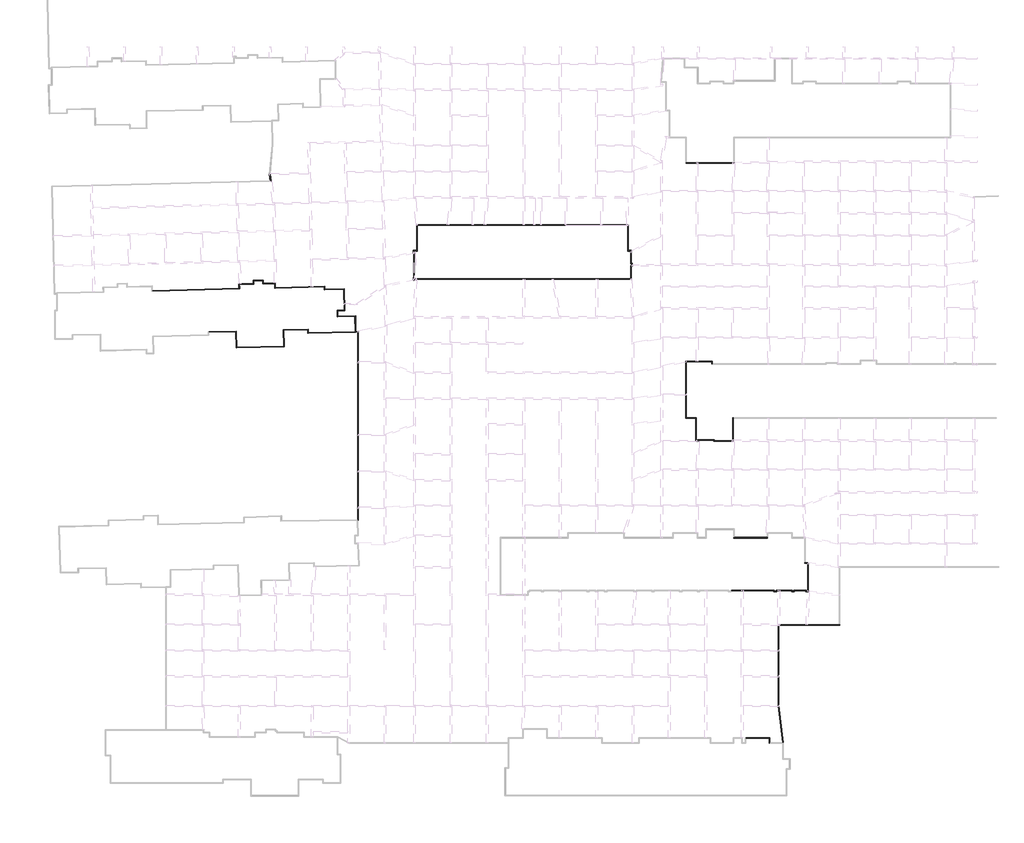
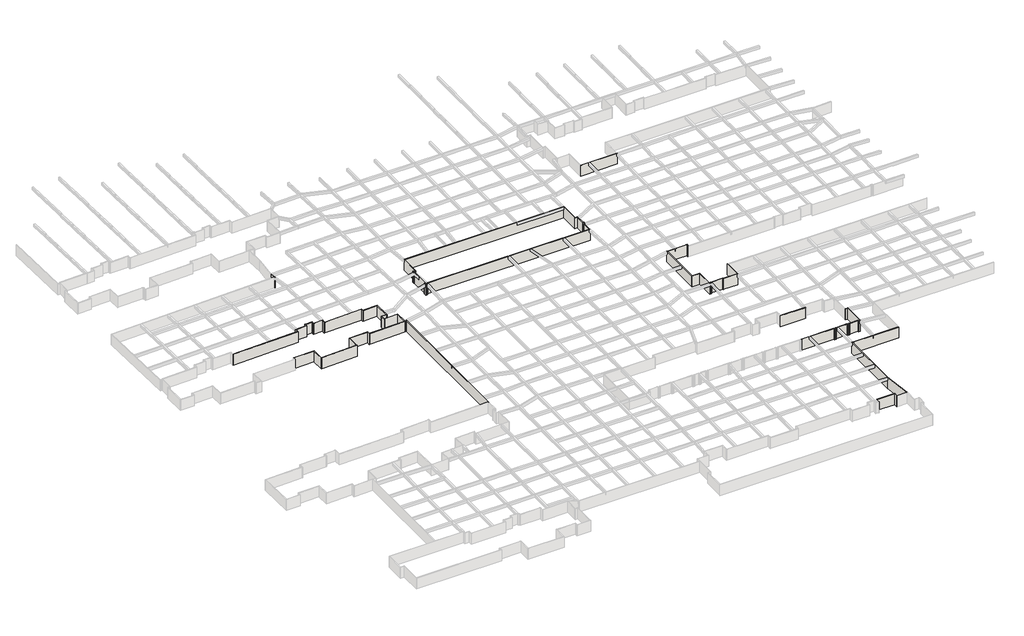
# One storey, part 4 of 20: 75 walls.
"""IFC4 building model written with IfcOpenShell, lengths in millimetres."""

from ifc_helpers import new_model, si_unit, origin, origin_with_axes, place, context, project, spatial, polyline, outline, extrude, faceted_brep, element, save

model = new_model("IFC4")

# Units and contexts
model_context = context("Model", 3, world=origin())
ifc_project = project(units=[si_unit("LENGTHUNIT", "METRE", prefix="MILLI")], contexts=[model_context])

# Site, building, storey
site = spatial("IfcSite", under=ifc_project)
building = spatial("IfcBuilding", under=site)
storey = spatial("IfcBuildingStorey", under=building, Name="户型图", Elevation=0.0)

# Walls
placement = place(None, origin())
element("IfcWall", 1, ObjectType="所有墙体", at=placement, inside=storey, context=model_context, shape_type="Brep", body=[
    faceted_brep([(22764.2529371, 124971.3529529, 0.0), (22969.277881, 123512.5246746, 0.0), (22986.0907128, 123392.8951605, 0.0), (22986.0907128, 123392.8951605, 3300.0), (22969.277881, 123512.5246746, 3300.0), (22764.2529371, 124971.3529529, 3300.0), (22884.987918, 124974.5145097, 0.0), (22884.987918, 124974.5145097, 3300.0), (23106.8607981, 123395.8069362, 3300.0), (23106.8607981, 123395.8069362, 0.0)], [[[0, 1, 2, 3, 4, 5]], [[6, 7, 8, 9]], [[2, 1, 0, 6, 9]], [[5, 4, 3, 8, 7]], [[0, 5, 7, 6]], [[3, 2, 9, 8]]]),
])
element("IfcWall", 2, ObjectType="所有墙体", at=placement, inside=storey, context=model_context, shape_type="Brep", body=[
    faceted_brep([(9470.1632227, 90251.8005582, 0.0), (15349.8840277, 90393.5386622, 0.0), (15469.8491762, 90396.4305738, 0.0), (15469.8491762, 90396.4305738, 3300.0), (15349.8840277, 90393.5386622, 3300.0), (9470.1632227, 90251.8005582, 3300.0), (9470.1632227, 90371.8354198, 0.0), (9470.1632227, 90371.8354198, 3300.0), (15466.9572646, 90516.3957223, 3300.0), (15466.9572646, 90516.3957223, 0.0)], [[[0, 1, 2, 3, 4, 5]], [[6, 7, 8, 9]], [[2, 1, 0, 6, 9]], [[5, 4, 3, 8, 7]], [[0, 5, 7, 6]], [[3, 2, 9, 8]]]),
])
element("IfcWall", 3, ObjectType="所有墙体", at=placement, inside=storey, context=model_context, shape_type="Brep", body=[
    faceted_brep([(15349.8840277, 90393.5386622, 0.0), (15435.7681225, 86830.8093449, 0.0), (15435.7681225, 86830.8093449, 3300.0), (15349.8840277, 90393.5386622, 3300.0), (15469.8491762, 90396.4305738, 0.0), (15469.8491762, 90396.4305738, 3300.0), (15552.8413594, 86953.6664049, 3300.0), (15555.7332709, 86833.7012564, 3300.0), (15555.7332709, 86833.7012564, 0.0), (15552.8413594, 86953.6664049, 0.0)], [[[0, 1, 2, 3]], [[4, 5, 6, 7, 8, 9]], [[1, 0, 4, 9, 8]], [[3, 2, 7, 6, 5]], [[0, 3, 5, 4]], [[2, 1, 8, 7]]]),
])
element("IfcWall", 4, ObjectType="所有墙体", at=placement, inside=storey, context=model_context, shape_type="Brep", body=[
    faceted_brep([(15555.7332709, 86833.7012564, 0.0), (25984.4133708, 87085.0977757, 0.0), (25984.4133708, 87085.0977757, 3300.0), (15555.7332709, 86833.7012564, 3300.0), (15552.8413594, 86953.6664049, 0.0), (15552.8413594, 86953.6664049, 3300.0), (25861.5563108, 87202.1710126, 3300.0), (25981.5214593, 87205.0629242, 3300.0), (25981.5214593, 87205.0629242, 0.0), (25861.5563108, 87202.1710126, 0.0)], [[[0, 1, 2, 3]], [[4, 5, 6, 7, 8, 9]], [[1, 0, 4, 9, 8]], [[3, 2, 7, 6, 5]], [[0, 3, 5, 4]], [[2, 1, 8, 7]]]),
])
element("IfcWall", 5, ObjectType="所有墙体", at=placement, inside=storey, context=model_context, shape_type="Brep", body=[
    faceted_brep([(25981.5214593, 87205.0629242, 0.0), (25898.5292761, 90647.8270931, 0.0), (25895.6373645, 90767.7922416, 0.0), (25895.6373645, 90767.7922416, 3300.0), (25898.5292761, 90647.8270931, 3300.0), (25981.5214593, 87205.0629242, 3300.0), (25861.5563108, 87202.1710126, 0.0), (25861.5563108, 87202.1710126, 3300.0), (25775.6722161, 90764.90033, 3300.0), (25775.6722161, 90764.90033, 0.0)], [[[0, 1, 2, 3, 4, 5]], [[6, 7, 8, 9]], [[2, 1, 0, 6, 9]], [[5, 4, 3, 8, 7]], [[0, 5, 7, 6]], [[3, 2, 9, 8]]]),
])
element("IfcWall", 6, ObjectType="所有墙体", at=placement, inside=storey, context=model_context, shape_type="Brep", body=[
    faceted_brep([(25898.5292761, 90647.8270931, 0.0), (31175.86669, 90775.0439838, 0.0), (31295.86669, 90777.9367356, 0.0), (31295.86669, 90777.9367356, 3300.0), (31175.86669, 90775.0439838, 3300.0), (25898.5292761, 90647.8270931, 3300.0), (25895.6373645, 90767.7922416, 0.0), (25895.6373645, 90767.7922416, 3300.0), (31295.86669, 90897.9715972, 3300.0), (31295.86669, 90897.9715972, 0.0)], [[[0, 1, 2, 3, 4, 5]], [[6, 7, 8, 9]], [[2, 1, 0, 6, 9]], [[5, 4, 3, 8, 7]], [[0, 5, 7, 6]], [[3, 2, 9, 8]]]),
])
element("IfcWall", 7, ObjectType="所有墙体", at=placement, inside=storey, context=model_context, shape_type="Brep", body=[
    faceted_brep([(31175.86669, 90775.0439838, 0.0), (31175.86669, 89975.0439838, 0.0), (31175.86669, 89975.0439838, 3300.0), (31175.86669, 90775.0439838, 3300.0), (31295.86669, 90777.9367356, 0.0), (31295.86669, 90777.9367356, 3300.0), (31295.86669, 90097.9715972, 3300.0), (31295.86669, 89977.9367356, 3300.0), (31295.86669, 89977.9367356, 0.0), (31295.86669, 90097.9715972, 0.0)], [[[0, 1, 2, 3]], [[4, 5, 6, 7, 8, 9]], [[1, 0, 4, 9, 8]], [[3, 2, 7, 6, 5]], [[0, 3, 5, 4]], [[2, 1, 8, 7]]]),
])
element("IfcWall", 8, ObjectType="所有墙体", at=placement, inside=storey, context=model_context, shape_type="SweptSolid", body=[
    extrude(outline(polyline([(41741.4257555, 90229.7401437), (31295.86669, 89977.9367356), (31295.86669, 90097.9715972), (41724.2086067, 90349.3599642), (41741.4257555, 90229.7401437)])), origin_with_axes(), (0.0, 0.0, 1.0), 3300.0),
])
element("IfcWall", 9, ObjectType="所有墙体", at=placement, inside=storey, context=model_context, shape_type="Brep", body=[
    faceted_brep([(41741.4257555, 90229.7401437, 0.0), (42190.0, 90349.9352502, 0.0), (42310.0, 90382.0891533, 0.0), (42310.0, 90382.0891533, 3300.0), (42190.0, 90349.9352502, 3300.0), (41741.4257555, 90229.7401437, 3300.0), (41724.2086067, 90349.3599642, 0.0), (41724.2086067, 90349.3599642, 3300.0), (42310.0, 90506.322295, 3300.0), (42310.0, 90506.322295, 0.0)], [[[0, 1, 2, 3, 4, 5]], [[6, 7, 8, 9]], [[2, 1, 0, 6, 9]], [[5, 4, 3, 8, 7]], [[0, 5, 7, 6]], [[3, 2, 9, 8]]]),
])
element("IfcWall", 10, ObjectType="所有墙体", at=placement, inside=storey, context=model_context, shape_type="Brep", body=[
    faceted_brep([(42190.0, 90349.9352502, 0.0), (42190.0, 49087.0906084, 0.0), (42190.0, 48967.072329, 0.0), (42190.0, 48967.072329, 3300.0), (42190.0, 49087.0906084, 3300.0), (42190.0, 90349.9352502, 3300.0), (42310.0, 90382.0891533, 0.0), (42310.0, 90382.0891533, 3300.0), (42310.0, 48969.1669368, 3300.0), (42310.0, 48969.1669368, 0.0)], [[[0, 1, 2, 3, 4, 5]], [[6, 7, 8, 9]], [[2, 1, 0, 6, 9]], [[5, 4, 3, 8, 7]], [[0, 5, 7, 6]], [[3, 2, 9, 8]]]),
])
element("IfcWall", 11, ObjectType="所有墙体", at=placement, inside=storey, context=model_context, shape_type="Brep", body=[
    faceted_brep([(127432.0, 1046.0, 0.0), (132562.0, 1046.0, 0.0), (132682.0, 1046.0, 0.0), (132682.0, 1046.0, 3300.0), (132562.0, 1046.0, 3300.0), (127432.0, 1046.0, 3300.0), (127432.0, 1166.0, 0.0), (127432.0, 1166.0, 3300.0), (132682.0, 1166.0, 3300.0), (132682.0, 1166.0, 0.0)], [[[0, 1, 2, 3, 4, 5]], [[6, 7, 8, 9]], [[2, 1, 0, 6, 9]], [[5, 4, 3, 8, 7]], [[0, 5, 7, 6]], [[3, 2, 9, 8]]]),
])
element("IfcWall", 12, ObjectType="所有墙体", at=placement, inside=storey, context=model_context, shape_type="Brep", body=[
    faceted_brep([(132562.0, 1046.0, 0.0), (132562.0, -63.5203758, 0.0), (132562.0, -63.5203758, 3300.0), (132562.0, 1046.0, 3300.0), (132682.0, 1046.0, 0.0), (132682.0, 1046.0, 3300.0), (132682.0, 56.4796242, 3300.0), (132682.0, -63.5203758, 3300.0), (132682.0, -63.5203758, 0.0), (132682.0, 56.4796242, 0.0)], [[[0, 1, 2, 3]], [[4, 5, 6, 7, 8, 9]], [[1, 0, 4, 9, 8]], [[3, 2, 7, 6, 5]], [[0, 3, 5, 4]], [[2, 1, 8, 7]]]),
])
element("IfcWall", 13, ObjectType="所有墙体", at=placement, inside=storey, context=model_context, shape_type="SweptSolid", body=[
    extrude(outline(polyline([(134683.7348611, 8238.28244), (135688.3339273, 56.4796242), (135567.4327482, 56.4796242), (134563.7348611, 8230.9429256), (134683.7348611, 8238.28244)])), origin_with_axes(), (0.0, 0.0, 1.0), 3300.0),
])
element("IfcWall", 14, ObjectType="所有墙体", at=placement, inside=storey, context=model_context, shape_type="Brep", body=[
    faceted_brep([(134683.7348611, 8238.28244, 0.0), (134683.7348611, 25874.6126828, 0.0), (134683.7348611, 25994.6126828, 0.0), (134683.7348611, 25994.6126828, 3300.0), (134683.7348611, 25874.6126828, 3300.0), (134683.7348611, 8238.28244, 3300.0), (134563.7348611, 8230.9429256, 0.0), (134563.7348611, 8230.9429256, 3300.0), (134563.7348611, 25994.6126828, 3300.0), (134563.7348611, 25994.6126828, 0.0)], [[[0, 1, 2, 3, 4, 5]], [[6, 7, 8, 9]], [[2, 1, 0, 6, 9]], [[5, 4, 3, 8, 7]], [[0, 5, 7, 6]], [[3, 2, 9, 8]]]),
])
element("IfcWall", 15, ObjectType="所有墙体", at=placement, inside=storey, context=model_context, shape_type="Brep", body=[
    faceted_brep([(134683.7348611, 25874.6126828, 0.0), (148100.0, 25874.6126828, 0.0), (148100.0, 25874.6126828, 3300.0), (134683.7348611, 25874.6126828, 3300.0), (134683.7348611, 25994.6126828, 0.0), (134683.7348611, 25994.6126828, 3300.0), (147980.0, 25994.6126828, 3300.0), (148100.0, 25994.6126828, 3300.0), (148100.0, 25994.6126828, 0.0), (147980.0, 25994.6126828, 0.0)], [[[0, 1, 2, 3]], [[4, 5, 6, 7, 8, 9]], [[1, 0, 4, 9, 8]], [[3, 2, 7, 6, 5]], [[0, 3, 5, 4]], [[2, 1, 8, 7]]]),
])
element("IfcWall", 16, ObjectType="所有墙体", at=placement, inside=storey, context=model_context, shape_type="Brep", body=[
    faceted_brep([(114310.0, 127379.0, 0.0), (124860.0, 127379.0, 0.0), (124860.0, 127379.0, 3300.0), (114310.0, 127379.0, 3300.0), (114310.0, 127499.0, 0.0), (114310.0, 127499.0, 3300.0), (124740.0, 127499.0, 3300.0), (124860.0, 127499.0, 3300.0), (124860.0, 127499.0, 0.0), (124740.0, 127499.0, 0.0)], [[[0, 1, 2, 3]], [[4, 5, 6, 7, 8, 9]], [[1, 0, 4, 9, 8]], [[3, 2, 7, 6, 5]], [[0, 3, 5, 4]], [[2, 1, 8, 7]]]),
])
element("IfcWall", 17, ObjectType="所有墙体", at=placement, inside=storey, context=model_context, shape_type="Brep", body=[
    faceted_brep([(114224.0, 83917.0, 0.0), (114224.0, 71310.0, 0.0), (114224.0, 71310.0, 3300.0), (114224.0, 83917.0, 3300.0), (114344.0, 83917.0, 0.0), (114344.0, 83917.0, 3300.0), (114344.0, 83797.0, 3300.0), (114344.0, 71430.0, 3300.0), (114344.0, 71310.0, 3300.0), (114344.0, 71310.0, 0.0), (114344.0, 71430.0, 0.0), (114344.0, 83797.0, 0.0)], [[[0, 1, 2, 3]], [[4, 5, 6, 7, 8, 9, 10, 11]], [[1, 0, 4, 11, 10, 9]], [[3, 2, 8, 7, 6, 5]], [[2, 1, 9, 8]], [[0, 3, 5, 4]]]),
])
element("IfcWall", 18, ObjectType="所有墙体", at=placement, inside=storey, context=model_context, shape_type="Brep", body=[
    faceted_brep([(114344.0, 71310.0, 0.0), (116431.0, 71310.0, 0.0), (116551.0, 71310.0, 0.0), (116551.0, 71310.0, 3300.0), (116431.0, 71310.0, 3300.0), (114344.0, 71310.0, 3300.0), (114344.0, 71430.0, 0.0), (114344.0, 71430.0, 3300.0), (116551.0, 71430.0, 3300.0), (116551.0, 71430.0, 0.0)], [[[0, 1, 2, 3, 4, 5]], [[6, 7, 8, 9]], [[2, 1, 0, 6, 9]], [[5, 4, 3, 8, 7]], [[0, 5, 7, 6]], [[3, 2, 9, 8]]]),
])
element("IfcWall", 19, ObjectType="所有墙体", at=placement, inside=storey, context=model_context, shape_type="Brep", body=[
    faceted_brep([(116431.0, 71310.0, 0.0), (116431.0, 66283.0, 0.0), (116431.0, 66283.0, 3300.0), (116431.0, 71310.0, 3300.0), (116551.0, 71310.0, 0.0), (116551.0, 71310.0, 3300.0), (116551.0, 66403.0, 3300.0), (116551.0, 66283.0, 3300.0), (116551.0, 66283.0, 0.0), (116551.0, 66403.0, 0.0)], [[[0, 1, 2, 3]], [[4, 5, 6, 7, 8, 9]], [[1, 0, 4, 9, 8]], [[3, 2, 7, 6, 5]], [[0, 3, 5, 4]], [[2, 1, 8, 7]]]),
])
element("IfcWall", 20, ObjectType="所有墙体", at=placement, inside=storey, context=model_context, shape_type="SweptSolid", body=[
    extrude(outline(polyline([(116917.0, 66283.0), (116551.0, 66283.0), (116551.0, 66403.0), (116917.0, 66403.0), (116917.0, 66283.0)])), origin_with_axes(), (0.0, 0.0, 1.0), 3300.0),
])
element("IfcWall", 21, ObjectType="所有墙体", at=placement, inside=storey, context=model_context, shape_type="Brep", body=[
    faceted_brep([(117037.0, 66283.0, 0.0), (117037.0, 66533.0, 0.0), (117037.0, 66653.0, 0.0), (117037.0, 66653.0, 3300.0), (117037.0, 66533.0, 3300.0), (117037.0, 66283.0, 3300.0), (116917.0, 66283.0, 0.0), (116917.0, 66283.0, 3300.0), (116917.0, 66403.0, 3300.0), (116917.0, 66653.0, 3300.0), (116917.0, 66653.0, 0.0), (116917.0, 66403.0, 0.0)], [[[0, 1, 2, 3, 4, 5]], [[6, 7, 8, 9, 10, 11]], [[2, 1, 0, 6, 11, 10]], [[5, 4, 3, 9, 8, 7]], [[0, 5, 7, 6]], [[3, 2, 10, 9]]]),
])
element("IfcWall", 22, ObjectType="所有墙体", at=placement, inside=storey, context=model_context, shape_type="SweptSolid", body=[
    extrude(outline(polyline([(120381.0, 66533.0), (117037.0, 66533.0), (117037.0, 66653.0), (120381.0, 66653.0), (120381.0, 66533.0)])), origin_with_axes(), (0.0, 0.0, 1.0), 3300.0),
])
element("IfcWall", 23, ObjectType="所有墙体", at=placement, inside=storey, context=model_context, shape_type="Brep", body=[
    faceted_brep([(120381.0, 66653.0, 0.0), (120381.0, 66533.0, 0.0), (120381.0, 66330.0, 0.0), (120381.0, 66330.0, 3300.0), (120381.0, 66533.0, 3300.0), (120381.0, 66653.0, 3300.0), (120501.0, 66653.0, 0.0), (120501.0, 66653.0, 3300.0), (120501.0, 66450.0, 3300.0), (120501.0, 66330.0, 3300.0), (120501.0, 66330.0, 0.0), (120501.0, 66450.0, 0.0)], [[[0, 1, 2, 3, 4, 5]], [[6, 7, 8, 9, 10, 11]], [[2, 1, 0, 6, 11, 10]], [[5, 4, 3, 9, 8, 7]], [[0, 5, 7, 6]], [[3, 2, 10, 9]]]),
])
element("IfcWall", 24, ObjectType="所有墙体", at=placement, inside=storey, context=model_context, shape_type="Brep", body=[
    faceted_brep([(120501.0, 66330.0, 0.0), (124710.0, 66330.0, 0.0), (124710.0, 66330.0, 3300.0), (120501.0, 66330.0, 3300.0), (120501.0, 66450.0, 0.0), (120501.0, 66450.0, 3300.0), (124590.0, 66450.0, 3300.0), (124710.0, 66450.0, 3300.0), (124710.0, 66450.0, 0.0), (124590.0, 66450.0, 0.0)], [[[0, 1, 2, 3]], [[4, 5, 6, 7, 8, 9]], [[1, 0, 4, 9, 8]], [[3, 2, 7, 6, 5]], [[0, 3, 5, 4]], [[2, 1, 8, 7]]]),
])
element("IfcWall", 25, ObjectType="所有墙体", at=placement, inside=storey, context=model_context, shape_type="Brep", body=[
    faceted_brep([(124710.0, 66450.0, 0.0), (124710.0, 71310.0, 0.0), (124710.0, 71430.0, 0.0), (124710.0, 71430.0, 3300.0), (124710.0, 71310.0, 3300.0), (124710.0, 66450.0, 3300.0), (124590.0, 66450.0, 0.0), (124590.0, 66450.0, 3300.0), (124590.0, 71430.0, 3300.0), (124590.0, 71430.0, 0.0)], [[[0, 1, 2, 3, 4, 5]], [[6, 7, 8, 9]], [[2, 1, 0, 6, 9]], [[5, 4, 3, 8, 7]], [[0, 5, 7, 6]], [[3, 2, 9, 8]]]),
])
element("IfcWall", 26, ObjectType="所有墙体", at=placement, inside=storey, context=model_context, shape_type="Brep", body=[
    faceted_brep([(120097.0, 83280.0, 0.0), (120097.0, 83917.0, 0.0), (120097.0, 83917.0, 3300.0), (120097.0, 83280.0, 3300.0), (119977.0, 83280.0, 0.0), (119977.0, 83280.0, 3300.0), (119977.0, 83797.0, 3300.0), (119977.0, 83917.0, 3300.0), (119977.0, 83917.0, 0.0), (119977.0, 83797.0, 0.0)], [[[0, 1, 2, 3]], [[4, 5, 6, 7, 8, 9]], [[1, 0, 4, 9, 8]], [[3, 2, 7, 6, 5]], [[0, 3, 5, 4]], [[2, 1, 8, 7]]]),
])
element("IfcWall", 27, ObjectType="所有墙体", at=placement, inside=storey, context=model_context, shape_type="SweptSolid", body=[
    extrude(outline(polyline([(114344.0, 83917.0), (119977.0, 83917.0), (119977.0, 83797.0), (114344.0, 83797.0), (114344.0, 83917.0)])), origin_with_axes(), (0.0, 0.0, 1.0), 3300.0),
])
element("IfcWall", 28, ObjectType="所有墙体", at=placement, inside=storey, context=model_context, shape_type="SweptSolid", body=[
    extrude(outline(polyline([(133584.0, 33447.0), (124204.0, 33447.0), (124204.0, 33567.0), (133584.0, 33567.0), (133584.0, 33447.0)])), origin_with_axes(), (0.0, 0.0, 1.0), 3300.0),
])
element("IfcWall", 29, ObjectType="所有墙体", at=placement, inside=storey, context=model_context, shape_type="Brep", body=[
    faceted_brep([(133584.0, 33567.0, 0.0), (133584.0, 33447.0, 0.0), (133584.0, 33197.0, 0.0), (133584.0, 33197.0, 3300.0), (133584.0, 33447.0, 3300.0), (133584.0, 33567.0, 3300.0), (133704.0, 33567.0, 0.0), (133704.0, 33567.0, 3300.0), (133704.0, 33317.0, 3300.0), (133704.0, 33197.0, 3300.0), (133704.0, 33197.0, 0.0), (133704.0, 33317.0, 0.0)], [[[0, 1, 2, 3, 4, 5]], [[6, 7, 8, 9, 10, 11]], [[2, 1, 0, 6, 11, 10]], [[5, 4, 3, 9, 8, 7]], [[0, 5, 7, 6]], [[3, 2, 10, 9]]]),
])
element("IfcWall", 30, ObjectType="所有墙体", at=placement, inside=storey, context=model_context, shape_type="SweptSolid", body=[
    extrude(outline(polyline([(134084.0, 33197.0), (133704.0, 33197.0), (133704.0, 33317.0), (134084.0, 33317.0), (134084.0, 33197.0)])), origin_with_axes(), (0.0, 0.0, 1.0), 3300.0),
])
element("IfcWall", 31, ObjectType="所有墙体", at=placement, inside=storey, context=model_context, shape_type="Brep", body=[
    faceted_brep([(134204.0, 33197.0, 0.0), (134204.0, 33447.0, 0.0), (134204.0, 33567.0, 0.0), (134204.0, 33567.0, 3300.0), (134204.0, 33447.0, 3300.0), (134204.0, 33197.0, 3300.0), (134084.0, 33197.0, 0.0), (134084.0, 33197.0, 3300.0), (134084.0, 33317.0, 3300.0), (134084.0, 33567.0, 3300.0), (134084.0, 33567.0, 0.0), (134084.0, 33317.0, 0.0)], [[[0, 1, 2, 3, 4, 5]], [[6, 7, 8, 9, 10, 11]], [[2, 1, 0, 6, 11, 10]], [[5, 4, 3, 9, 8, 7]], [[0, 5, 7, 6]], [[3, 2, 10, 9]]]),
])
element("IfcWall", 32, ObjectType="所有墙体", at=placement, inside=storey, context=model_context, shape_type="SweptSolid", body=[
    extrude(outline(polyline([(137484.0, 33447.0), (134204.0, 33447.0), (134204.0, 33567.0), (137484.0, 33567.0), (137484.0, 33447.0)])), origin_with_axes(), (0.0, 0.0, 1.0), 3300.0),
])
element("IfcWall", 33, ObjectType="所有墙体", at=placement, inside=storey, context=model_context, shape_type="Brep", body=[
    faceted_brep([(137484.0, 33567.0, 0.0), (137484.0, 33447.0, 0.0), (137484.0, 33197.0, 0.0), (137484.0, 33197.0, 3300.0), (137484.0, 33447.0, 3300.0), (137484.0, 33567.0, 3300.0), (137604.0, 33567.0, 0.0), (137604.0, 33567.0, 3300.0), (137604.0, 33317.0, 3300.0), (137604.0, 33197.0, 3300.0), (137604.0, 33197.0, 0.0), (137604.0, 33317.0, 0.0)], [[[0, 1, 2, 3, 4, 5]], [[6, 7, 8, 9, 10, 11]], [[2, 1, 0, 6, 11, 10]], [[5, 4, 3, 9, 8, 7]], [[0, 5, 7, 6]], [[3, 2, 10, 9]]]),
])
element("IfcWall", 34, ObjectType="所有墙体", at=placement, inside=storey, context=model_context, shape_type="SweptSolid", body=[
    extrude(outline(polyline([(137984.0, 33197.0), (137604.0, 33197.0), (137604.0, 33317.0), (137984.0, 33317.0), (137984.0, 33197.0)])), origin_with_axes(), (0.0, 0.0, 1.0), 3300.0),
])
element("IfcWall", 35, ObjectType="所有墙体", at=placement, inside=storey, context=model_context, shape_type="Brep", body=[
    faceted_brep([(138104.0, 33197.0, 0.0), (138104.0, 33447.0, 0.0), (138104.0, 33567.0, 0.0), (138104.0, 33567.0, 3300.0), (138104.0, 33447.0, 3300.0), (138104.0, 33197.0, 3300.0), (137984.0, 33197.0, 0.0), (137984.0, 33197.0, 3300.0), (137984.0, 33317.0, 3300.0), (137984.0, 33567.0, 3300.0), (137984.0, 33567.0, 0.0), (137984.0, 33317.0, 0.0)], [[[0, 1, 2, 3, 4, 5]], [[6, 7, 8, 9, 10, 11]], [[2, 1, 0, 6, 11, 10]], [[5, 4, 3, 9, 8, 7]], [[0, 5, 7, 6]], [[3, 2, 10, 9]]]),
])
element("IfcWall", 36, ObjectType="所有墙体", at=placement, inside=storey, context=model_context, shape_type="SweptSolid", body=[
    extrude(outline(polyline([(140584.0, 33447.0), (138104.0, 33447.0), (138104.0, 33567.0), (140584.0, 33567.0), (140584.0, 33447.0)])), origin_with_axes(), (0.0, 0.0, 1.0), 3300.0),
])
element("IfcWall", 37, ObjectType="所有墙体", at=placement, inside=storey, context=model_context, shape_type="Brep", body=[
    faceted_brep([(140584.0, 33567.0, 0.0), (140584.0, 33447.0, 0.0), (140584.0, 33197.0, 0.0), (140584.0, 33197.0, 3300.0), (140584.0, 33447.0, 3300.0), (140584.0, 33567.0, 3300.0), (140704.0, 33567.0, 0.0), (140704.0, 33567.0, 3300.0), (140704.0, 33317.0, 3300.0), (140704.0, 33197.0, 3300.0), (140704.0, 33197.0, 0.0), (140704.0, 33317.0, 0.0)], [[[0, 1, 2, 3, 4, 5]], [[6, 7, 8, 9, 10, 11]], [[2, 1, 0, 6, 11, 10]], [[5, 4, 3, 9, 8, 7]], [[0, 5, 7, 6]], [[3, 2, 10, 9]]]),
])
element("IfcWall", 38, ObjectType="所有墙体", at=placement, inside=storey, context=model_context, shape_type="Brep", body=[
    faceted_brep([(140704.0, 33197.0, 0.0), (141192.159458, 33197.0, 0.0), (141192.159458, 33197.0, 3300.0), (140704.0, 33197.0, 3300.0), (140704.0, 33317.0, 0.0), (140704.0, 33317.0, 3300.0), (141072.159458, 33317.0, 3300.0), (141192.159458, 33317.0, 3300.0), (141192.159458, 33317.0, 0.0), (141072.159458, 33317.0, 0.0)], [[[0, 1, 2, 3]], [[4, 5, 6, 7, 8, 9]], [[1, 0, 4, 9, 8]], [[3, 2, 7, 6, 5]], [[0, 3, 5, 4]], [[2, 1, 8, 7]]]),
])
element("IfcWall", 39, ObjectType="所有墙体", at=placement, inside=storey, context=model_context, shape_type="Brep", body=[
    faceted_brep([(141192.159458, 33317.0, 0.0), (141192.159458, 39568.0, 0.0), (141192.159458, 39568.0, 3300.0), (141192.159458, 33317.0, 3300.0), (141072.159458, 33317.0, 0.0), (141072.159458, 33317.0, 3300.0), (141072.159458, 39448.0, 3300.0), (141072.159458, 39568.0, 3300.0), (141072.159458, 39568.0, 0.0), (141072.159458, 39448.0, 0.0)], [[[0, 1, 2, 3]], [[4, 5, 6, 7, 8, 9]], [[1, 0, 4, 9, 8]], [[3, 2, 7, 6, 5]], [[0, 3, 5, 4]], [[2, 1, 8, 7]]]),
])
element("IfcWall", 40, ObjectType="所有墙体", at=placement, inside=storey, context=model_context, shape_type="Brep", body=[
    faceted_brep([(141072.159458, 39568.0, 0.0), (140504.0, 39568.0, 0.0), (140384.0, 39568.0, 0.0), (140384.0, 39568.0, 3300.0), (140504.0, 39568.0, 3300.0), (141072.159458, 39568.0, 3300.0), (141072.159458, 39448.0, 0.0), (141072.159458, 39448.0, 3300.0), (140384.0, 39448.0, 3300.0), (140384.0, 39448.0, 0.0)], [[[0, 1, 2, 3, 4, 5]], [[6, 7, 8, 9]], [[2, 1, 0, 6, 9]], [[5, 4, 3, 8, 7]], [[0, 5, 7, 6]], [[3, 2, 9, 8]]]),
])
element("IfcWall", 41, ObjectType="所有墙体", at=placement, inside=storey, context=model_context, shape_type="Brep", body=[
    faceted_brep([(132088.0, 45158.2500378, 0.0), (124911.0, 45158.2500378, 0.0), (124791.0, 45158.2500378, 0.0), (124791.0, 45158.2500378, 3300.0), (124911.0, 45158.2500378, 3300.0), (132088.0, 45158.2500378, 3300.0), (132088.0, 45038.2500378, 0.0), (132088.0, 45038.2500378, 3300.0), (124791.0, 45038.2500378, 3300.0), (124791.0, 45038.2500378, 0.0)], [[[0, 1, 2, 3, 4, 5]], [[6, 7, 8, 9]], [[2, 1, 0, 6, 9]], [[5, 4, 3, 8, 7]], [[0, 5, 7, 6]], [[3, 2, 9, 8]]]),
])
element("IfcWall", 42, ObjectType="所有墙体", at=placement, inside=storey, context=model_context, shape_type="Brep", body=[
    faceted_brep([(-2967.4697531, 99291.4669416, 0.0), (16186.957102, 99753.5620098, 0.0), (16186.957102, 99753.5620098, 3300.0), (-2967.4697531, 99291.4669416, 3300.0), (-2970.3638767, 99411.4320367, 0.0), (-2970.3638767, 99411.4320367, 3300.0), (16064.0978833, 99870.6329813, 3300.0), (16184.0629784, 99873.5271049, 3300.0), (16184.0629784, 99873.5271049, 0.0), (16064.0978833, 99870.6329813, 0.0)], [[[0, 1, 2, 3]], [[4, 5, 6, 7, 8, 9]], [[1, 0, 4, 9, 8]], [[3, 2, 7, 6, 5]], [[0, 3, 5, 4]], [[2, 1, 8, 7]]]),
])
element("IfcWall", 43, ObjectType="所有墙体", at=placement, inside=storey, context=model_context, shape_type="Brep", body=[
    faceted_brep([(16184.0629784, 99873.5271049, 0.0), (16162.8529382, 100752.7101819, 0.0), (16159.9588146, 100872.675277, 0.0), (16159.9588146, 100872.675277, 3300.0), (16162.8529382, 100752.7101819, 3300.0), (16184.0629784, 99873.5271049, 3300.0), (16064.0978833, 99870.6329813, 0.0), (16064.0978833, 99870.6329813, 3300.0), (16039.9937195, 100869.7811534, 3300.0), (16039.9937195, 100869.7811534, 0.0)], [[[0, 1, 2, 3, 4, 5]], [[6, 7, 8, 9]], [[2, 1, 0, 6, 9]], [[5, 4, 3, 8, 7]], [[0, 5, 7, 6]], [[3, 2, 9, 8]]]),
])
element("IfcWall", 44, ObjectType="所有墙体", at=placement, inside=storey, context=model_context, shape_type="Brep", body=[
    faceted_brep([(16162.8529382, 100752.7101819, 0.0), (19299.9780023, 100828.3924266, 0.0), (19299.9780023, 100828.3924266, 3300.0), (16162.8529382, 100752.7101819, 3300.0), (16159.9588146, 100872.675277, 0.0), (16159.9588146, 100872.675277, 3300.0), (19179.9780023, 100945.532376, 3300.0), (19299.9780023, 100948.4273417, 3300.0), (19299.9780023, 100948.4273417, 0.0), (19179.9780023, 100945.532376, 0.0)], [[[0, 1, 2, 3]], [[4, 5, 6, 7, 8, 9]], [[1, 0, 4, 9, 8]], [[3, 2, 7, 6, 5]], [[0, 3, 5, 4]], [[2, 1, 8, 7]]]),
])
element("IfcWall", 45, ObjectType="所有墙体", at=placement, inside=storey, context=model_context, shape_type="Brep", body=[
    faceted_brep([(19299.9780023, 100948.4273417, 0.0), (19299.9780023, 101528.3924266, 0.0), (19299.9780023, 101648.4273417, 0.0), (19299.9780023, 101648.4273417, 3300.0), (19299.9780023, 101528.3924266, 3300.0), (19299.9780023, 100948.4273417, 3300.0), (19179.9780023, 100945.532376, 0.0), (19179.9780023, 100945.532376, 3300.0), (19179.9780023, 101645.532376, 3300.0), (19179.9780023, 101645.532376, 0.0)], [[[0, 1, 2, 3, 4, 5]], [[6, 7, 8, 9]], [[2, 1, 0, 6, 9]], [[5, 4, 3, 8, 7]], [[0, 5, 7, 6]], [[3, 2, 9, 8]]]),
])
element("IfcWall", 46, ObjectType="所有墙体", at=placement, inside=storey, context=model_context, shape_type="Brep", body=[
    faceted_brep([(19299.9780023, 101528.3924266, 0.0), (21260.8374987, 101575.697601, 0.0), (21380.8025938, 101578.5917246, 0.0), (21380.8025938, 101578.5917246, 3300.0), (21260.8374987, 101575.697601, 3300.0), (19299.9780023, 101528.3924266, 3300.0), (19299.9780023, 101648.4273417, 0.0), (19299.9780023, 101648.4273417, 3300.0), (21377.9084702, 101698.5568197, 3300.0), (21377.9084702, 101698.5568197, 0.0)], [[[0, 1, 2, 3, 4, 5]], [[6, 7, 8, 9]], [[2, 1, 0, 6, 9]], [[5, 4, 3, 8, 7]], [[0, 5, 7, 6]], [[3, 2, 9, 8]]]),
])
element("IfcWall", 47, ObjectType="所有墙体", at=placement, inside=storey, context=model_context, shape_type="Brep", body=[
    faceted_brep([(21260.8374987, 101575.697601, 0.0), (21277.7149757, 100876.1047653, 0.0), (21277.7149757, 100876.1047653, 3300.0), (21260.8374987, 101575.697601, 3300.0), (21380.8025938, 101578.5917246, 0.0), (21380.8025938, 101578.5917246, 3300.0), (21394.7859472, 100998.963984, 3300.0), (21397.6800708, 100878.9988889, 3300.0), (21397.6800708, 100878.9988889, 0.0), (21394.7859472, 100998.963984, 0.0)], [[[0, 1, 2, 3]], [[4, 5, 6, 7, 8, 9]], [[1, 0, 4, 9, 8]], [[3, 2, 7, 6, 5]], [[0, 3, 5, 4]], [[2, 1, 8, 7]]]),
])
element("IfcWall", 48, ObjectType="所有墙体", at=placement, inside=storey, context=model_context, shape_type="Brep", body=[
    faceted_brep([(21397.6800708, 100878.9988889, 0.0), (23929.002874, 100940.0663274, 0.0), (24049.002874, 100942.9612931, 0.0), (24049.002874, 100942.9612931, 3300.0), (23929.002874, 100940.0663274, 3300.0), (21397.6800708, 100878.9988889, 3300.0), (21394.7859472, 100998.963984, 0.0), (21394.7859472, 100998.963984, 3300.0), (24049.002874, 101062.9962081, 3300.0), (24049.002874, 101062.9962081, 0.0)], [[[0, 1, 2, 3, 4, 5]], [[6, 7, 8, 9]], [[2, 1, 0, 6, 9]], [[5, 4, 3, 8, 7]], [[0, 5, 7, 6]], [[3, 2, 9, 8]]]),
])
element("IfcWall", 49, ObjectType="所有墙体", at=placement, inside=storey, context=model_context, shape_type="Brep", body=[
    faceted_brep([(23929.002874, 100940.0663274, 0.0), (23929.002874, 99940.0663274, 0.0), (23929.002874, 99940.0663274, 3300.0), (23929.002874, 100940.0663274, 3300.0), (24049.002874, 100942.9612931, 0.0), (24049.002874, 100942.9612931, 3300.0), (24049.002874, 100062.9962081, 3300.0), (24049.002874, 99942.9612931, 3300.0), (24049.002874, 99942.9612931, 0.0), (24049.002874, 100062.9962081, 0.0)], [[[0, 1, 2, 3]], [[4, 5, 6, 7, 8, 9]], [[1, 0, 4, 9, 8]], [[3, 2, 7, 6, 5]], [[0, 3, 5, 4]], [[2, 1, 8, 7]]]),
])
element("IfcWall", 50, ObjectType="所有墙体", at=placement, inside=storey, context=model_context, shape_type="Brep", body=[
    faceted_brep([(24049.002874, 99942.9612931, 0.0), (34825.832348, 100202.9492211, 0.0), (34945.832348, 100205.8441868, 0.0), (34945.832348, 100205.8441868, 3300.0), (34825.832348, 100202.9492211, 3300.0), (24049.002874, 99942.9612931, 3300.0), (24049.002874, 100062.9962081, 0.0), (24049.002874, 100062.9962081, 3300.0), (34945.832348, 100325.8791018, 3300.0), (34945.832348, 100325.8791018, 0.0)], [[[0, 1, 2, 3, 4, 5]], [[6, 7, 8, 9]], [[2, 1, 0, 6, 9]], [[5, 4, 3, 8, 7]], [[0, 5, 7, 6]], [[3, 2, 9, 8]]]),
])
element("IfcWall", 51, ObjectType="所有墙体", at=placement, inside=storey, context=model_context, shape_type="Brep", body=[
    faceted_brep([(34825.832348, 100202.9492211, 0.0), (34825.832348, 99602.9492211, 0.0), (34825.832348, 99602.9492211, 3300.0), (34825.832348, 100202.9492211, 3300.0), (34945.832348, 100205.8441868, 0.0), (34945.832348, 100205.8441868, 3300.0), (34945.832348, 99725.8791018, 3300.0), (34945.832348, 99605.8441868, 3300.0), (34945.832348, 99605.8441868, 0.0), (34945.832348, 99725.8791018, 0.0)], [[[0, 1, 2, 3]], [[4, 5, 6, 7, 8, 9]], [[1, 0, 4, 9, 8]], [[3, 2, 7, 6, 5]], [[0, 3, 5, 4]], [[2, 1, 8, 7]]]),
])
element("IfcWall", 52, ObjectType="所有墙体", at=placement, inside=storey, context=model_context, shape_type="Brep", body=[
    faceted_brep([(34945.832348, 99605.8441868, 0.0), (39046.0693741, 99704.761232, 0.0), (39166.0344693, 99707.6553556, 0.0), (39166.0344693, 99707.6553556, 3300.0), (39046.0693741, 99704.761232, 3300.0), (34945.832348, 99605.8441868, 3300.0), (34945.832348, 99725.8791018, 0.0), (34945.832348, 99725.8791018, 3300.0), (39163.1403457, 99827.6204507, 3300.0), (39163.1403457, 99827.6204507, 0.0)], [[[0, 1, 2, 3, 4, 5]], [[6, 7, 8, 9]], [[2, 1, 0, 6, 9]], [[5, 4, 3, 8, 7]], [[0, 5, 7, 6]], [[3, 2, 9, 8]]]),
])
element("IfcWall", 53, ObjectType="所有墙体", at=placement, inside=storey, context=model_context, shape_type="Brep", body=[
    faceted_brep([(39046.0693741, 99704.761232, 0.0), (39156.576379, 95124.105674, 0.0), (39159.4705026, 95004.1405789, 0.0), (39159.4705026, 95004.1405789, 3300.0), (39156.576379, 95124.105674, 3300.0), (39046.0693741, 99704.761232, 3300.0), (39166.0344693, 99707.6553556, 0.0), (39166.0344693, 99707.6553556, 3300.0), (39279.4355978, 95007.0347025, 3300.0), (39279.4355978, 95007.0347025, 0.0)], [[[0, 1, 2, 3, 4, 5]], [[6, 7, 8, 9]], [[2, 1, 0, 6, 9]], [[5, 4, 3, 8, 7]], [[0, 5, 7, 6]], [[3, 2, 9, 8]]]),
])
element("IfcWall", 54, ObjectType="所有墙体", at=placement, inside=storey, context=model_context, shape_type="Brep", body=[
    faceted_brep([(39156.576379, 95124.105674, 0.0), (37625.5790869, 95087.1708023, 0.0), (37625.5790869, 95087.1708023, 3300.0), (39156.576379, 95124.105674, 3300.0), (39159.4705026, 95004.1405789, 0.0), (39159.4705026, 95004.1405789, 3300.0), (37748.4383057, 94970.0998308, 3300.0), (37628.4732105, 94967.2057072, 3300.0), (37628.4732105, 94967.2057072, 0.0), (37748.4383057, 94970.0998308, 0.0)], [[[0, 1, 2, 3]], [[4, 5, 6, 7, 8, 9]], [[1, 0, 4, 9, 8]], [[3, 2, 7, 6, 5]], [[0, 3, 5, 4]], [[2, 1, 8, 7]]]),
])
element("IfcWall", 55, ObjectType="所有墙体", at=placement, inside=storey, context=model_context, shape_type="Brep", body=[
    faceted_brep([(37628.4732105, 94967.2057072, 0.0), (37659.8263303, 93667.5791136, 0.0), (37659.8263303, 93667.5791136, 3300.0), (37628.4732105, 94967.2057072, 3300.0), (37748.4383057, 94970.0998308, 0.0), (37748.4383057, 94970.0998308, 3300.0), (37776.8973018, 93790.4383323, 3300.0), (37779.7914254, 93670.4732372, 3300.0), (37779.7914254, 93670.4732372, 0.0), (37776.8973018, 93790.4383323, 0.0)], [[[0, 1, 2, 3]], [[4, 5, 6, 7, 8, 9]], [[1, 0, 4, 9, 8]], [[3, 2, 7, 6, 5]], [[0, 3, 5, 4]], [[2, 1, 8, 7]]]),
])
element("IfcWall", 56, ObjectType="所有墙体", at=placement, inside=storey, context=model_context, shape_type="Brep", body=[
    faceted_brep([(37779.7914254, 93670.4732372, 0.0), (41558.4619146, 93761.6325817, 0.0), (41678.4270097, 93764.5267053, 0.0), (41678.4270097, 93764.5267053, 3300.0), (41558.4619146, 93761.6325817, 3300.0), (37779.7914254, 93670.4732372, 3300.0), (37776.8973018, 93790.4383323, 0.0), (37776.8973018, 93790.4383323, 3300.0), (41675.5350981, 93884.4918538, 3300.0), (41675.5350981, 93884.4918538, 0.0)], [[[0, 1, 2, 3, 4, 5]], [[6, 7, 8, 9]], [[2, 1, 0, 6, 9]], [[5, 4, 3, 8, 7]], [[0, 5, 7, 6]], [[3, 2, 9, 8]]]),
])
element("IfcWall", 57, ObjectType="所有墙体", at=placement, inside=storey, context=model_context, shape_type="SweptSolid", body=[
    extrude(outline(polyline([(41640.7675489, 90347.348512), (41558.4619146, 93761.6325817), (41678.4270097, 93764.5267053), (41760.5193814, 90359.089407), (41724.2086067, 90349.3599642), (41640.7675489, 90347.348512)])), origin_with_axes(), (0.0, 0.0, 1.0), 3300.0),
])
element("IfcWall", 58, ObjectType="所有墙体", at=placement, inside=storey, context=model_context, shape_type="Brep", body=[
    faceted_brep([(55098.0, 113857.0, 0.0), (55098.0, 108206.0, 0.0), (55098.0, 108086.0, 0.0), (55098.0, 108086.0, 3300.0), (55098.0, 108206.0, 3300.0), (55098.0, 113857.0, 3300.0), (55218.0, 113857.0, 0.0), (55218.0, 113857.0, 3300.0), (55218.0, 113737.0, 3300.0), (55218.0, 108086.0, 3300.0), (55218.0, 108086.0, 0.0), (55218.0, 113737.0, 0.0)], [[[0, 1, 2, 3, 4, 5]], [[6, 7, 8, 9, 10, 11]], [[2, 1, 0, 6, 11, 10]], [[5, 4, 3, 9, 8, 7]], [[3, 2, 10, 9]], [[0, 5, 7, 6]]]),
])
element("IfcWall", 59, ObjectType="所有墙体", at=placement, inside=storey, context=model_context, shape_type="Brep", body=[
    faceted_brep([(55098.0, 108206.0, 0.0), (54340.0, 108206.0, 0.0), (54340.0, 108206.0, 3300.0), (55098.0, 108206.0, 3300.0), (55098.0, 108086.0, 0.0), (55098.0, 108086.0, 3300.0), (54460.0, 108086.0, 3300.0), (54340.0, 108086.0, 3300.0), (54340.0, 108086.0, 0.0), (54460.0, 108086.0, 0.0)], [[[0, 1, 2, 3]], [[4, 5, 6, 7, 8, 9]], [[1, 0, 4, 9, 8]], [[3, 2, 7, 6, 5]], [[0, 3, 5, 4]], [[2, 1, 8, 7]]]),
])
element("IfcWall", 60, ObjectType="所有墙体", at=placement, inside=storey, context=model_context, shape_type="SweptSolid", body=[
    extrude(outline(polyline([(54340.0, 107706.0), (54340.0, 108086.0), (54460.0, 108086.0), (54460.0, 107706.0), (54340.0, 107706.0)])), origin_with_axes(), (0.0, 0.0, 1.0), 3300.0),
])
element("IfcWall", 61, ObjectType="所有墙体", at=placement, inside=storey, context=model_context, shape_type="Brep", body=[
    faceted_brep([(54340.0, 107586.0, 0.0), (54498.0, 107586.0, 0.0), (54618.0, 107586.0, 0.0), (54618.0, 107586.0, 3300.0), (54498.0, 107586.0, 3300.0), (54340.0, 107586.0, 3300.0), (54340.0, 107706.0, 0.0), (54340.0, 107706.0, 3300.0), (54460.0, 107706.0, 3300.0), (54618.0, 107706.0, 3300.0), (54618.0, 107706.0, 0.0), (54460.0, 107706.0, 0.0)], [[[0, 1, 2, 3, 4, 5]], [[6, 7, 8, 9, 10, 11]], [[2, 1, 0, 6, 11, 10]], [[5, 4, 3, 9, 8, 7]], [[0, 5, 7, 6]], [[3, 2, 10, 9]]]),
])
element("IfcWall", 62, ObjectType="所有墙体", at=placement, inside=storey, context=model_context, shape_type="SweptSolid", body=[
    extrude(outline(polyline([(54498.0, 102256.0), (54498.0, 107586.0), (54618.0, 107586.0), (54618.0, 102256.0), (54498.0, 102256.0)])), origin_with_axes(), (0.0, 0.0, 1.0), 3300.0),
])
element("IfcWall", 63, ObjectType="所有墙体", at=placement, inside=storey, context=model_context, shape_type="Brep", body=[
    faceted_brep([(54618.0, 102256.0, 0.0), (54498.0, 102256.0, 0.0), (54340.0, 102256.0, 0.0), (54340.0, 102256.0, 3300.0), (54498.0, 102256.0, 3300.0), (54618.0, 102256.0, 3300.0), (54618.0, 102136.0, 0.0), (54618.0, 102136.0, 3300.0), (54460.0, 102136.0, 3300.0), (54340.0, 102136.0, 3300.0), (54340.0, 102136.0, 0.0), (54460.0, 102136.0, 0.0)], [[[0, 1, 2, 3, 4, 5]], [[6, 7, 8, 9, 10, 11]], [[2, 1, 0, 6, 11, 10]], [[5, 4, 3, 9, 8, 7]], [[0, 5, 7, 6]], [[3, 2, 10, 9]]]),
])
element("IfcWall", 64, ObjectType="所有墙体", at=placement, inside=storey, context=model_context, shape_type="Brep", body=[
    faceted_brep([(54340.0, 102136.0, 0.0), (54340.0, 101636.0, 0.0), (54340.0, 101636.0, 2500.0), (54340.0, 101636.0, 3300.0), (54340.0, 102006.0, 3300.0), (54340.0, 102136.0, 3300.0), (54460.0, 102136.0, 0.0), (54460.0, 102136.0, 3300.0), (54460.0, 102006.0, 3300.0), (54460.0, 101756.0, 3300.0), (54460.0, 101636.0, 3300.0), (54460.0, 101636.0, 0.0), (54460.0, 101756.0, 0.0), (54435.4694471, 101636.0, 3300.0)], [[[0, 1, 2, 3, 4, 5]], [[6, 7, 8, 9, 10, 11, 12]], [[1, 0, 6, 12, 11]], [[5, 4, 3, 13, 10, 9, 8, 7]], [[0, 5, 7, 6]], [[3, 2, 1, 11, 10, 13]]]),
])
element("IfcWall", 65, ObjectType="所有墙体", at=placement, inside=storey, context=model_context, shape_type="Brep", body=[
    faceted_brep([(54460.0, 101636.0, 0.0), (54840.0, 101636.0, 0.0), (54840.0, 101636.0, 3300.0), (54690.7253782, 101636.0, 3300.0), (54460.0, 101636.0, 3300.0), (54460.0, 101756.0, 0.0), (54460.0, 101756.0, 3300.0), (54694.2815659, 101756.0, 3300.0), (54840.0, 101756.0, 3300.0), (54840.0, 101756.0, 2500.0), (54840.0, 101756.0, 0.0)], [[[0, 1, 2, 3, 4]], [[5, 6, 7, 8, 9, 10]], [[1, 0, 5, 10]], [[4, 3, 2, 8, 7, 6]], [[0, 4, 6, 5]], [[2, 1, 10, 9, 8]]]),
])
element("IfcWall", 66, ObjectType="所有墙体", at=placement, inside=storey, context=model_context, shape_type="Brep", body=[
    faceted_brep([(54960.0, 101636.0, 0.0), (54960.0, 101886.0, 0.0), (54960.0, 102006.0, 0.0), (54960.0, 102006.0, 3300.0), (54960.0, 101886.0, 3300.0), (54960.0, 101636.0, 3300.0), (54840.0, 101636.0, 0.0), (54840.0, 101636.0, 3300.0), (54840.0, 101756.0, 3300.0), (54840.0, 102006.0, 3300.0), (54840.0, 102006.0, 0.0), (54840.0, 101756.0, 0.0)], [[[0, 1, 2, 3, 4, 5]], [[6, 7, 8, 9, 10, 11]], [[2, 1, 0, 6, 11, 10]], [[5, 4, 3, 9, 8, 7]], [[0, 5, 7, 6]], [[3, 2, 10, 9]]]),
])
element("IfcWall", 67, ObjectType="所有墙体", at=placement, inside=storey, context=model_context, shape_type="Brep", body=[
    faceted_brep([(54960.0, 101886.0, 0.0), (102249.0, 101886.0, 0.0), (102249.0, 101886.0, 3300.0), (54960.0, 101886.0, 3300.0), (54960.0, 102006.0, 0.0), (54960.0, 102006.0, 3300.0), (102129.0, 102006.0, 3300.0), (102249.0, 102006.0, 3300.0), (102249.0, 102006.0, 0.0), (102129.0, 102006.0, 0.0)], [[[0, 1, 2, 3]], [[4, 5, 6, 7, 8, 9]], [[1, 0, 4, 9, 8]], [[3, 2, 7, 6, 5]], [[0, 3, 5, 4]], [[2, 1, 8, 7]]]),
])
element("IfcWall", 68, ObjectType="所有墙体", at=placement, inside=storey, context=model_context, shape_type="SweptSolid", body=[
    extrude(outline(polyline([(102249.0, 104780.0), (102249.0, 102006.0), (102129.0, 102006.0), (102129.0, 104780.0), (102249.0, 104780.0)])), origin_with_axes(), (0.0, 0.0, 1.0), 3300.0),
])
element("IfcWall", 69, ObjectType="所有墙体", at=placement, inside=storey, context=model_context, shape_type="Brep", body=[
    faceted_brep([(102129.0, 104780.0, 0.0), (102249.0, 104780.0, 0.0), (102514.0, 104780.0, 0.0), (102514.0, 104780.0, 3300.0), (102249.0, 104780.0, 3300.0), (102129.0, 104780.0, 3300.0), (102129.0, 104900.0, 0.0), (102129.0, 104900.0, 3300.0), (102394.0, 104900.0, 3300.0), (102514.0, 104900.0, 3300.0), (102514.0, 104900.0, 0.0), (102394.0, 104900.0, 0.0)], [[[0, 1, 2, 3, 4, 5]], [[6, 7, 8, 9, 10, 11]], [[2, 1, 0, 6, 11, 10]], [[5, 4, 3, 9, 8, 7]], [[0, 5, 7, 6]], [[3, 2, 10, 9]]]),
])
element("IfcWall", 70, ObjectType="所有墙体", at=placement, inside=storey, context=model_context, shape_type="SweptSolid", body=[
    extrude(outline(polyline([(102514.0, 105280.0), (102514.0, 104900.0), (102394.0, 104900.0), (102394.0, 105280.0), (102514.0, 105280.0)])), origin_with_axes(), (0.0, 0.0, 1.0), 3300.0),
])
element("IfcWall", 71, ObjectType="所有墙体", at=placement, inside=storey, context=model_context, shape_type="Brep", body=[
    faceted_brep([(102514.0, 105400.0, 0.0), (102249.0, 105400.0, 0.0), (102129.0, 105400.0, 0.0), (102129.0, 105400.0, 3300.0), (102249.0, 105400.0, 3300.0), (102514.0, 105400.0, 3300.0), (102514.0, 105280.0, 0.0), (102514.0, 105280.0, 3300.0), (102394.0, 105280.0, 3300.0), (102129.0, 105280.0, 3300.0), (102129.0, 105280.0, 0.0), (102394.0, 105280.0, 0.0)], [[[0, 1, 2, 3, 4, 5]], [[6, 7, 8, 9, 10, 11]], [[2, 1, 0, 6, 11, 10]], [[5, 4, 3, 9, 8, 7]], [[0, 5, 7, 6]], [[3, 2, 10, 9]]]),
])
element("IfcWall", 72, ObjectType="所有墙体", at=placement, inside=storey, context=model_context, shape_type="Brep", body=[
    faceted_brep([(102249.0, 105400.0, 0.0), (102249.0, 108207.0, 0.0), (102249.0, 108207.0, 3300.0), (102249.0, 105400.0, 3300.0), (102129.0, 105400.0, 0.0), (102129.0, 105400.0, 3300.0), (102129.0, 108087.0, 3300.0), (102129.0, 108207.0, 3300.0), (102129.0, 108207.0, 0.0), (102129.0, 108087.0, 0.0)], [[[0, 1, 2, 3]], [[4, 5, 6, 7, 8, 9]], [[1, 0, 4, 9, 8]], [[3, 2, 7, 6, 5]], [[0, 3, 5, 4]], [[2, 1, 8, 7]]]),
])
element("IfcWall", 73, ObjectType="所有墙体", at=placement, inside=storey, context=model_context, shape_type="Brep", body=[
    faceted_brep([(102129.0, 108207.0, 0.0), (101564.0, 108207.0, 0.0), (101444.0, 108207.0, 0.0), (101444.0, 108207.0, 3300.0), (101564.0, 108207.0, 3300.0), (102129.0, 108207.0, 3300.0), (102129.0, 108087.0, 0.0), (102129.0, 108087.0, 3300.0), (101444.0, 108087.0, 3300.0), (101444.0, 108087.0, 0.0)], [[[0, 1, 2, 3, 4, 5]], [[6, 7, 8, 9]], [[2, 1, 0, 6, 9]], [[5, 4, 3, 8, 7]], [[0, 5, 7, 6]], [[3, 2, 9, 8]]]),
])
element("IfcWall", 74, ObjectType="所有墙体", at=placement, inside=storey, context=model_context, shape_type="Brep", body=[
    faceted_brep([(101564.0, 108207.0, 0.0), (101564.0, 113857.0, 0.0), (101564.0, 113857.0, 3300.0), (101564.0, 108207.0, 3300.0), (101444.0, 108207.0, 0.0), (101444.0, 108207.0, 3300.0), (101444.0, 113737.0, 3300.0), (101444.0, 113857.0, 3300.0), (101444.0, 113857.0, 0.0), (101444.0, 113737.0, 0.0)], [[[0, 1, 2, 3]], [[4, 5, 6, 7, 8, 9]], [[1, 0, 4, 9, 8]], [[3, 2, 7, 6, 5]], [[0, 3, 5, 4]], [[2, 1, 8, 7]]]),
])
element("IfcWall", 75, ObjectType="所有墙体", at=placement, inside=storey, context=model_context, shape_type="Brep", body=[
    faceted_brep([(101444.0, 113857.0, 0.0), (55218.0, 113857.0, 0.0), (55218.0, 113857.0, 3300.0), (87904.0, 113857.0, 3300.0), (95604.0, 113857.0, 3300.0), (95804.0, 113857.0, 3300.0), (101301.782845, 113857.0, 3300.0), (101444.0, 113857.0, 3300.0), (101444.0, 113737.0, 0.0), (101444.0, 113737.0, 2500.0), (101444.0, 113737.0, 3300.0), (95804.0, 113737.0, 3300.0), (87904.0, 113737.0, 3300.0), (55218.0, 113737.0, 3300.0), (55218.0, 113737.0, 0.0)], [[[0, 1, 2, 3, 4, 5, 6, 7]], [[8, 9, 10, 11, 12, 13, 14]], [[1, 0, 8, 14]], [[7, 6, 5, 4, 3, 2, 13, 12, 11, 10]], [[2, 1, 14, 13]], [[0, 7, 10, 9, 8]]]),
])

save(model, "model.ifc")

# Revit data of these elements
# Type "所有墙体"
#   Layers, outside or top first: 120 mm "默认" (function 1)
# Elements 1, 2, 3, 4, 5, 6, 7, 8, 9, 10, 11, 12, 13, 14, 15, 16, 17, 18, 19, 20, 21, 22, 23, 24, 25, 26, 27, 28, 29, 30, 31, 32, 33, 34, 35, 36, 37, 38, 39, 40, 41 (IfcWall, "所有墙体")
#   Top Offset = 0 mm
#   Base Offset = 0 mm
#   wall height = 3300 mm
#   Phase Created = 新构造
#   Base Constraint = 户型图
#   Top Constraint = 层高
#   Materials on its faces: "默认"
# Elements 42, 43, 44, 45, 46, 47, 48, 49, 50, 51, 52, 53, 54, 55, 56, 57, 58, 59, 60, 61, 62, 63, 64, 65, 66, 67, 68, 69, 70, 71, 72, 73, 74, 75 (IfcWall, "所有墙体")
#   Comments = ""
#   Top Offset = 0 mm
#   Base Offset = 0 mm
#   wall height = 3300 mm
#   Phase Created = 新构造
#   Base Constraint = 户型图
#   Top Constraint = 层高
#   Materials on its faces: "默认"
# Materials
#   "默认": class "其他", colour RGB 192 192 192, transparency 0, Cost = 0
